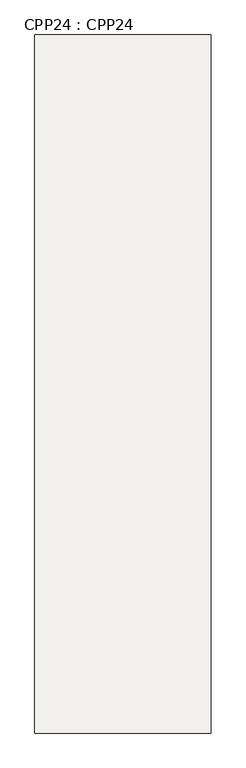
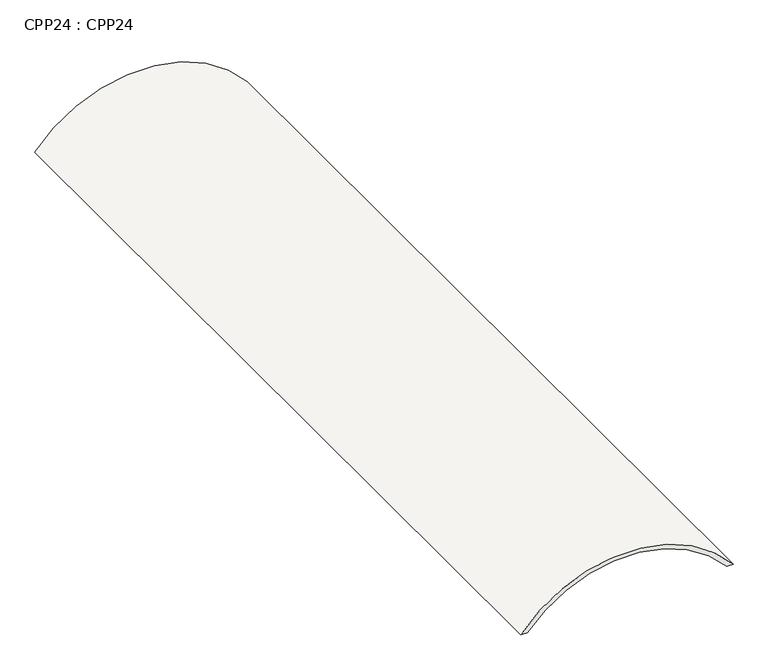
"""IFC4 building model written with IfcOpenShell, lengths in millimetres: slab geometry, CPP24 : CPP24."""

from ifc_helpers import new_model, si_unit, point, frame, frame_2d, origin, place, context, project, spatial, polyline, circle_curve, trimmed, segment, composite_curve, outline, extrude, source, transform, mapped, element, save


def cpp24_cpp24_22fb0938(model_context):
    return source(origin(), model_context, "Body", "SweptSolid", [
        extrude(outline(composite_curve([segment(polyline([(14620.0, 30333.2245515), (14620.0, 30483.2245515)]), True, "CONTINUOUS"), segment(trimmed(circle_curve(frame_2d((12603.2870371, 32833.2245514)), 3096.7129629), [point((14620.0, 30483.2245515))], [point((14620.0, 35183.2245514))], True, "CARTESIAN"), True, "CONTINUOUS"), segment(polyline([(14620.0, 35183.2245514), (14620.0, 35333.2245514)]), True, "CONTINUOUS"), segment(trimmed(circle_curve(frame_2d((12561.6949153, 32833.2245514)), 3238.3050847), [point((14620.0, 35333.2245514))], [point((14620.0, 30333.2245515))], False, "CARTESIAN"), True, "CONTINUOUS")], self_intersect=False)), frame((0.0, -100.2551788, 0.0), z_axis=(0.0, 1.0, 0.0), x_axis=(0.0, 0.0, 1.0)), (0.0, 0.0, 1.0), 19800.2551781),
    ])


if __name__ == "__main__":
    model = new_model("IFC4")
    model_context = context("Model", 3, world=origin())
    ifc_project = project(units=[si_unit("LENGTHUNIT", "METRE", prefix="MILLI")], contexts=[model_context])
    site = spatial("IfcSite", under=ifc_project)
    building = spatial("IfcBuilding", under=site)
    placement = place(None, origin())
    cpp24_cpp24_shape = cpp24_cpp24_22fb0938(model_context)
    element("IfcSlab", 1, ObjectType="CPP24 : CPP24", at=placement, inside=building, context=model_context, shape_type="MappedRepresentation", body=[
        mapped(cpp24_cpp24_shape, transform((0.0, 0.0, 0.0), x_axis=(1.0, 0.0, 0.0), y_axis=(0.0, 1.0, 0.0), z_axis=(0.0, 0.0, 1.0))),
    ])
    save(model, "model.ifc")

# Revit data of these elements
# Element 1 (IfcSlab, "CPP24 : CPP24")
#   Materials on its faces: "Concrete, RC"
# Materials
#   "Concrete, RC": class "Concrete", colour RGB 128 128 128, transparency 0, Description = "Cast-in-place concrete", Cost = 0
